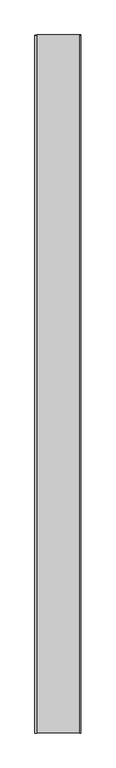
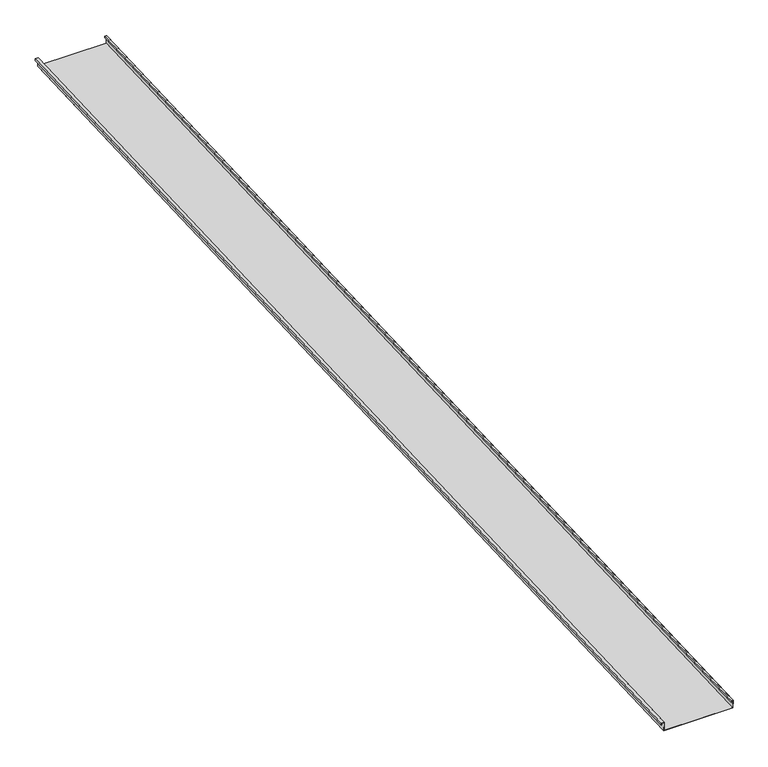
"""IFC4 building model written with IfcOpenShell, lengths in millimetres: proxy geometry, Generic Models 2:Generic Models 2:310765:Generic Models 2:310765 : Generic Models 2:Generic Models 2:310765:127 : Generic Models 2:Generic Models 2:310765:Generic Models 2:310765 : Generic Models 2:Generic Models 2:310765:300385."""

from ifc_helpers import new_model, si_unit, frame, origin, place, context, project, spatial, polyline, outline, extrude, source, transform, mapped, element, save


def generic_models_81f1c45a(model_context):
    return source(origin(), model_context, "Body", "SweptSolid", [
        extrude(outline(polyline([(1.5875, 0.0), (1.5875, 50.8), (407.9875, 50.8), (407.9875, 1.5875), (396.875, 1.5875), (396.875, 11.1125), (398.4625, 11.1125), (398.4625, 3.175), (406.4, 3.175), (406.4, 49.2125), (3.175, 49.2125), (3.175, -1.5874999), (-14.2875, -1.5874999), (-14.2875, 9.525), (-12.7, 9.525), (-12.7, 0.0), (1.5875, 0.0)])), frame((661758.4929738, -581354.4345603, 3902.6697972), z_axis=(0.0, 0.9991330730923568, 0.041630544712067834), x_axis=(1.0, 0.0, 0.0)), (0.0, 0.0, 1.0), 6400.8),
    ])


if __name__ == "__main__":
    model = new_model("IFC4")
    model_context = context("Model", 3, world=origin())
    ifc_project = project(units=[si_unit("LENGTHUNIT", "METRE", prefix="MILLI")], contexts=[model_context])
    site = spatial("IfcSite", under=ifc_project)
    building = spatial("IfcBuilding", under=site)
    placement = place(None, origin())
    generic_models_shape = generic_models_81f1c45a(model_context)
    element("IfcBuildingElementProxy", 1, Name="Generic Models 2:Generic Models 2:310765:Generic Models 2:310765 : Generic Models 2:Generic Models 2:310765:127 : Generic Models 2:Generic Models 2:310765:Generic Models 2:310765 : Generic Models 2:Generic Models 2:310765:300385", ObjectType="Generic Models 2:Generic Models 2:310765:Generic Models 2:310765 : Generic Models 2:Generic Models 2:310765:127 : Generic Models 2:Generic Models 2:310765:Generic Models 2:310765 : Generic Models 2:Generic Models 2:310765:300385", at=placement, inside=building, context=model_context, shape_type="MappedRepresentation", body=[
        mapped(generic_models_shape, transform((0.0, 0.0, 0.0), x_axis=(1.0, 0.0, 0.0), y_axis=(0.0, 1.0, 0.0), z_axis=(0.0, 0.0, 1.0))),
    ])
    save(model, "model.ifc")

# Revit data of these elements
# Type "Generic Models 2:Generic Models 2:310765:Generic Models 2:310765 : Generic Models 2:Generic Models 2:310765:127 : Generic Models 2:Generic Models 2:310765:Generic Models 2:310765 : Generic Models 2:Generic Models 2:310765:300385"
#   NameOverride = "Generic Models 2:Generic Models 2:310765:Generic Models 2:310765 : Generic Models 2:Generic Models 2:310765:300385"
#   ObjectTypeOverride = "Generic Models 2:310765 : Generic Models 2:Generic Models 2:310765"
#   Reference = "Generic Models 2"
#   Tag = "300385"
# Element 1 (IfcBuildingElementProxy, "Generic Models 2:Generic Models 2:310765:Generic Models 2:310765 : Generic Models 2:Generic Models 2:310765:127 : Generic Models 2:Generic Models 2:310765:Generic Models 2:310765 : Generic Models 2:Generic Models 2:310765:300385")
#   Materials on its faces: "THERMAL BROKEN ALUMINUM STOREFRONT FOR POLYCARBONATE"
# Materials
#   "THERMAL BROKEN ALUMINUM STOREFRONT FOR POLYCARBONATE": class "Unassigned", colour RGB 244 244 244, transparency 0, Keynote = "M07611300.01", Cost = 0
